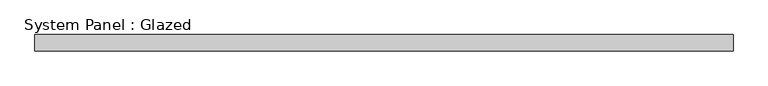
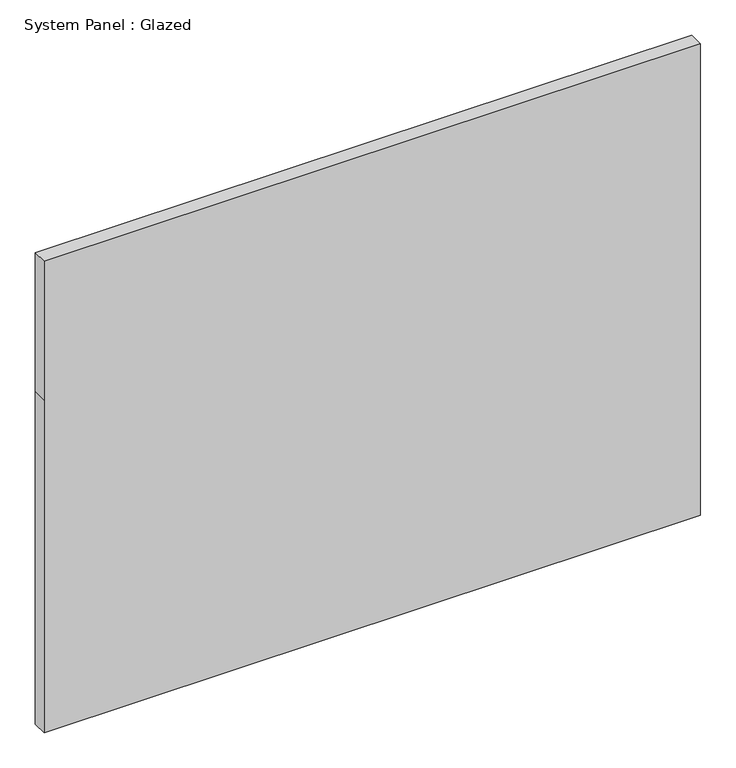
"""IFC4 building model written with IfcOpenShell, lengths in millimetres: plate geometry, System Panel : Glazed."""

from ifc_helpers import new_model, si_unit, frame, origin, place, context, project, spatial, polyline, outline, extrude, source, transform, mapped, element, save


def system_panel_glazed_0463a73c(model_context):
    return source(origin(), model_context, "Body", "SweptSolid", [
        extrude(outline(polyline([(0.0, -539.3822881), (0.0, 539.3822881), (577.85, 539.3822881), (819.15, 539.3822881), (819.15, -539.3822881), (577.85, -539.3822881), (0.0, -539.3822881)])), frame((0.0, -44.45, 0.0), z_axis=(0.0, 1.0, 0.0), x_axis=(0.0, 0.0, 1.0)), (0.0, 0.0, 1.0), 25.4),
    ])


if __name__ == "__main__":
    model = new_model("IFC4")
    model_context = context("Model", 3, world=origin())
    ifc_project = project(units=[si_unit("LENGTHUNIT", "METRE", prefix="MILLI")], contexts=[model_context])
    site = spatial("IfcSite", under=ifc_project)
    building = spatial("IfcBuilding", under=site)
    placement = place(None, origin())
    system_panel_glazed_shape = system_panel_glazed_0463a73c(model_context)
    element("IfcPlate", 1, ObjectType="System Panel : Glazed", at=placement, inside=building, context=model_context, shape_type="MappedRepresentation", body=[
        mapped(system_panel_glazed_shape, transform((0.0, 0.0, 0.0), x_axis=(1.0, 0.0, 0.0), y_axis=(0.0, 1.0, 0.0), z_axis=(0.0, 0.0, 1.0))),
    ])
    save(model, "model.ifc")

# Revit data of these elements
# Project information
#   SR Document GUID = "d36f5d78-752a-40d6-a009-b379f065f3eb"
# Element 1 (IfcPlate, "System Panel : Glazed")
#   Materials on its faces: "Glass"
# Materials
#   "Glass": class "Unassigned", colour RGB 147 173 200, transparency 0.7, Cost = 0
